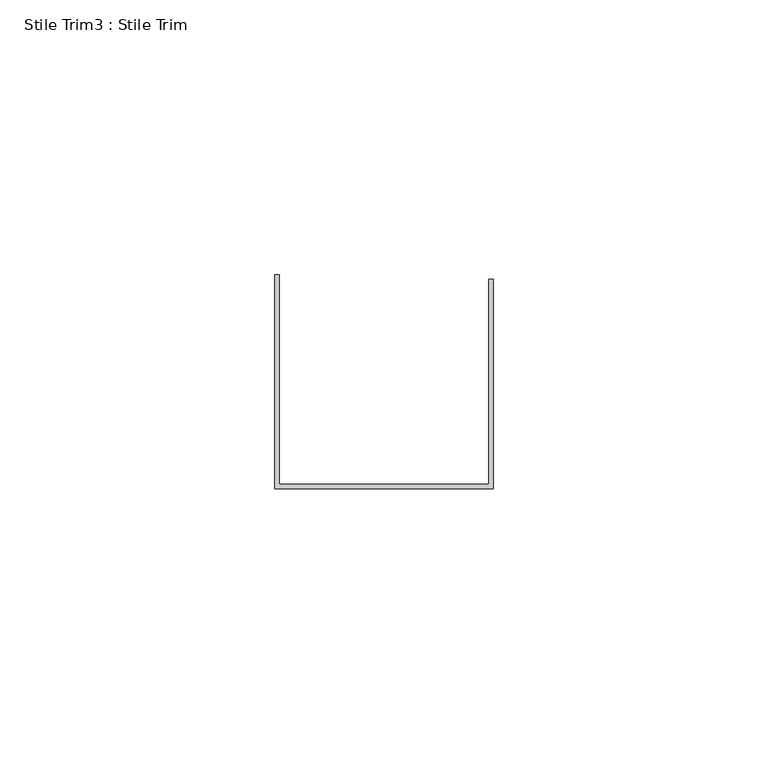
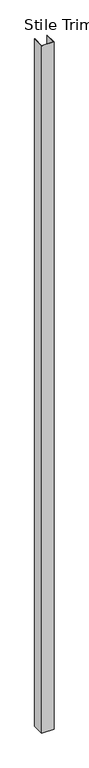
"""IFC4 building model written with IfcOpenShell, lengths in millimetres: proxy geometry, Stile Trim3 : Stile Trim."""

from ifc_helpers import new_model, si_unit, frame, origin, place, context, project, spatial, polyline, outline, extrude, source, transform, mapped, element, save


def stile_trim3_stile_trim_de7d98ae(model_context):
    return source(origin(), model_context, "Body", "SweptSolid", [
        extrude(outline(polyline([(587327.0060739, -533978.3912841), (587327.0060739, -533939.5038841), (587327.7934739, -533939.5038841), (587327.7934739, -533977.6038841), (587365.8934739, -533977.6038841), (587365.8934739, -533940.2912841), (587366.6808739, -533940.2912841), (587366.6808739, -533978.3912841), (587327.0060739, -533978.3912841)])), frame((0.0, 0.0, 50.8), z_axis=(0.0, 0.0, 1.0), x_axis=(1.0, 0.0, 0.0)), (0.0, 0.0, 1.0), 2350.3929688),
    ])


if __name__ == "__main__":
    model = new_model("IFC4")
    model_context = context("Model", 3, world=origin())
    ifc_project = project(units=[si_unit("LENGTHUNIT", "METRE", prefix="MILLI")], contexts=[model_context])
    site = spatial("IfcSite", under=ifc_project)
    building = spatial("IfcBuilding", under=site)
    placement = place(None, origin())
    stile_trim3_stile_trim_shape = stile_trim3_stile_trim_de7d98ae(model_context)
    element("IfcBuildingElementProxy", 1, Name="Stile Trim3 : Stile Trim", ObjectType="Stile Trim3 : Stile Trim", at=placement, inside=building, context=model_context, shape_type="MappedRepresentation", body=[
        mapped(stile_trim3_stile_trim_shape, transform((0.0, 0.0, 0.0), x_axis=(1.0, 0.0, 0.0), y_axis=(0.0, 1.0, 0.0), z_axis=(0.0, 0.0, 1.0))),
    ])
    save(model, "model.ifc")

# Revit data of these elements
# Element 1 (IfcBuildingElementProxy, "Stile Trim3 : Stile Trim")
#   Materials on its faces: "EDGE TRIM BY MTL PANEL MFR."
# Materials
#   "EDGE TRIM BY MTL PANEL MFR.": class "Generic", colour RGB 239 242 240, transparency 0, Cost = 0
